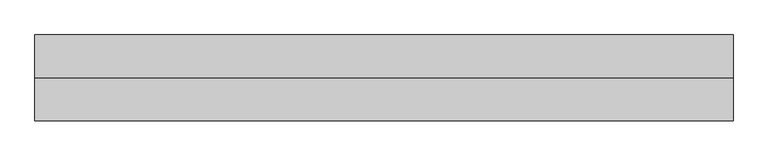
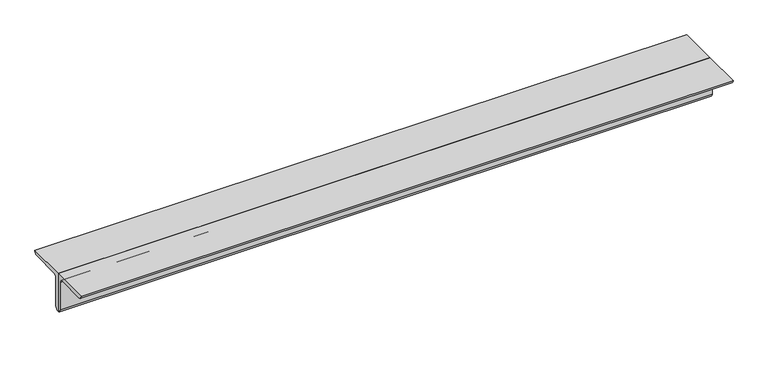
"""IFC4 building model written with IfcOpenShell, lengths in millimetres: beam geometry, 0123_Steel Framing_2Ls-KSD3502 : H_SB_AR_S04_2Ls-130x130x12_VBR1."""

from ifc_helpers import new_model, si_unit, point, frame, frame_2d, origin, place, context, project, spatial, polyline, circle_curve, trimmed, segment, composite_curve, outline, extrude, source, transform, mapped, element, save


def beam_893a5a9c(model_context):
    return source(origin(), model_context, "Body", "SweptSolid", [
        extrude(outline(composite_curve([segment(polyline([(0.0, 36.4), (130.0, 36.4)]), True, "CONTINUOUS"), segment(trimmed(circle_curve(frame_2d((118.0, 36.4)), 12.0), [point((130.0, 36.4))], [point((118.0, 24.4))], False, "CARTESIAN"), True, "CONTINUOUS"), segment(polyline([(118.0, 24.4), (24.0, 24.4)]), True, "CONTINUOUS"), segment(trimmed(circle_curve(frame_2d((24.0, 12.4)), 12.0), [point((24.0, 24.4))], [point((12.0, 12.4))], True, "CARTESIAN"), True, "CONTINUOUS"), segment(polyline([(12.0, 12.4), (12.0, -81.6)]), True, "CONTINUOUS"), segment(trimmed(circle_curve(frame_2d((0.0, -81.6)), 12.0), [point((12.0, -81.6))], [point((0.0, -93.6))], False, "CARTESIAN"), True, "CONTINUOUS"), segment(polyline([(0.0, -93.6), (0.0, 36.4)]), True, "CONTINUOUS")], self_intersect=False)), frame((-991.4315887, 0.0, 0.0), z_axis=(1.0, 0.0, 0.0), x_axis=(0.0, 1.0, 0.0)), (0.0, 0.0, 1.0), 2118.004285),
        extrude(outline(composite_curve([segment(polyline([(0.0, 36.4), (0.0, -93.6)]), True, "CONTINUOUS"), segment(trimmed(circle_curve(frame_2d((0.0, -81.6)), 12.0), [point((0.0, -93.6))], [point((-12.0, -81.6))], False, "CARTESIAN"), True, "CONTINUOUS"), segment(polyline([(-12.0, -81.6), (-12.0, 12.4)]), True, "CONTINUOUS"), segment(trimmed(circle_curve(frame_2d((-24.0, 12.4)), 12.0), [point((-12.0, 12.4))], [point((-24.0, 24.4))], True, "CARTESIAN"), True, "CONTINUOUS"), segment(polyline([(-24.0, 24.4), (-118.0, 24.4)]), True, "CONTINUOUS"), segment(trimmed(circle_curve(frame_2d((-118.0, 36.4)), 12.0), [point((-118.0, 24.4))], [point((-130.0, 36.4))], False, "CARTESIAN"), True, "CONTINUOUS"), segment(polyline([(-130.0, 36.4), (0.0, 36.4)]), True, "CONTINUOUS")], self_intersect=False)), frame((-991.4315887, 0.0, 0.0), z_axis=(1.0, 0.0, 0.0), x_axis=(0.0, 1.0, 0.0)), (0.0, 0.0, 1.0), 2118.004285),
    ])


if __name__ == "__main__":
    model = new_model("IFC4")
    model_context = context("Model", 3, world=origin())
    ifc_project = project(units=[si_unit("LENGTHUNIT", "METRE", prefix="MILLI")], contexts=[model_context])
    site = spatial("IfcSite", under=ifc_project)
    building = spatial("IfcBuilding", under=site)
    placement = place(None, origin())
    beam_shape = beam_893a5a9c(model_context)
    element("IfcBeam", 1, ObjectType="0123_Steel Framing_2Ls-KSD3502 : H_SB_AR_S04_2Ls-130x130x12_VBR1", at=placement, inside=building, context=model_context, shape_type="MappedRepresentation", body=[
        mapped(beam_shape, transform((0.0, 0.0, 0.0), x_axis=(1.0, 0.0, 0.0), y_axis=(0.0, 1.0, 0.0), z_axis=(0.0, 0.0, 1.0))),
    ])
    save(model, "model.ifc")

# Revit data of these elements
# Type "0123_Steel Framing_2Ls-KSD3502 : H_SB_AR_S04_2Ls-130x130x12_VBR1"
#   Type Mark = "VBR1"
#   Assembly Code = "B10"
#   Legs = "SLBB"
#   W = 8.97
#   Perimeter = 1.04 m²/m
#   Nominal Weight = 46.80 kgf/m
#   Length [instance default] = 1000 mm
#   Space = 0 mm
#   b = 130 mm
#   d = 130 mm
#   t = 12 mm
#   y = 36.4 mm
#   A = 0.005952 m²
#   Structural Material [instance default] = Steel ASTM A36
# Element 1 (IfcBeam, "0123_Steel Framing_2Ls-KSD3502 : H_SB_AR_S04_2Ls-130x130x12_VBR1")
#   Materials on its faces: "Steel ASTM A36"
# Materials
#   "Steel ASTM A36": class "Metal", colour RGB 199 199 199, transparency 0, Description = "Structural steel, ASTM A36 Grade B, mill finish", Cost = 0
